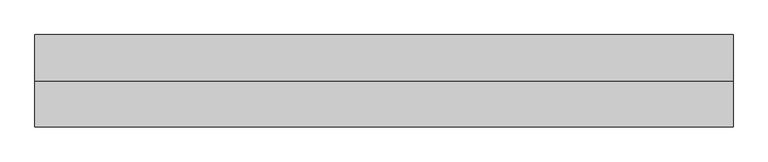
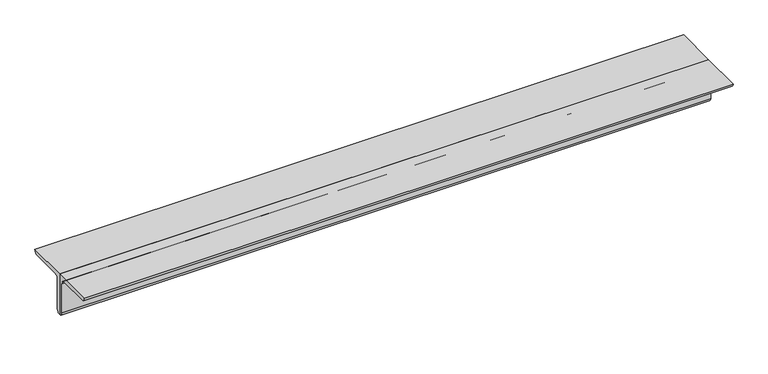
"""IFC4 building model written with IfcOpenShell, lengths in millimetres: beam geometry, 0123_Steel Framing_2Ls-KSD3502 : H_SB_AR_S04_2Ls-130x130x12_VBR1."""

from ifc_helpers import new_model, si_unit, point, frame, frame_2d, origin, place, context, project, spatial, polyline, circle_curve, trimmed, segment, composite_curve, outline, extrude, source, transform, mapped, element, save


def beam_0ae2001c(model_context):
    return source(origin(), model_context, "Body", "SweptSolid", [
        extrude(outline(composite_curve([segment(polyline([(0.0, 36.4), (130.0, 36.4)]), True, "CONTINUOUS"), segment(trimmed(circle_curve(frame_2d((118.0, 36.4)), 12.0), [point((130.0, 36.4))], [point((118.0, 24.4))], False, "CARTESIAN"), True, "CONTINUOUS"), segment(polyline([(118.0, 24.4), (24.0, 24.4)]), True, "CONTINUOUS"), segment(trimmed(circle_curve(frame_2d((24.0, 12.4)), 12.0), [point((24.0, 24.4))], [point((12.0, 12.4))], True, "CARTESIAN"), True, "CONTINUOUS"), segment(polyline([(12.0, 12.4), (12.0, -81.6)]), True, "CONTINUOUS"), segment(trimmed(circle_curve(frame_2d((0.0, -81.6)), 12.0), [point((12.0, -81.6))], [point((0.0, -93.6))], False, "CARTESIAN"), True, "CONTINUOUS"), segment(polyline([(0.0, -93.6), (0.0, 36.4)]), True, "CONTINUOUS")], self_intersect=False)), frame((-912.8215992, 0.0, 0.0), z_axis=(1.0, 0.0, 0.0), x_axis=(0.0, 1.0, 0.0)), (0.0, 0.0, 1.0), 1965.6424176),
        extrude(outline(composite_curve([segment(polyline([(0.0, 36.4), (0.0, -93.6)]), True, "CONTINUOUS"), segment(trimmed(circle_curve(frame_2d((0.0, -81.6)), 12.0), [point((0.0, -93.6))], [point((-12.0, -81.6))], False, "CARTESIAN"), True, "CONTINUOUS"), segment(polyline([(-12.0, -81.6), (-12.0, 12.4)]), True, "CONTINUOUS"), segment(trimmed(circle_curve(frame_2d((-24.0, 12.4)), 12.0), [point((-12.0, 12.4))], [point((-24.0, 24.4))], True, "CARTESIAN"), True, "CONTINUOUS"), segment(polyline([(-24.0, 24.4), (-118.0, 24.4)]), True, "CONTINUOUS"), segment(trimmed(circle_curve(frame_2d((-118.0, 36.4)), 12.0), [point((-118.0, 24.4))], [point((-130.0, 36.4))], False, "CARTESIAN"), True, "CONTINUOUS"), segment(polyline([(-130.0, 36.4), (0.0, 36.4)]), True, "CONTINUOUS")], self_intersect=False)), frame((-912.8215992, 0.0, 0.0), z_axis=(1.0, 0.0, 0.0), x_axis=(0.0, 1.0, 0.0)), (0.0, 0.0, 1.0), 1965.6424176),
    ])


if __name__ == "__main__":
    model = new_model("IFC4")
    model_context = context("Model", 3, world=origin())
    ifc_project = project(units=[si_unit("LENGTHUNIT", "METRE", prefix="MILLI")], contexts=[model_context])
    site = spatial("IfcSite", under=ifc_project)
    building = spatial("IfcBuilding", under=site)
    placement = place(None, origin())
    beam_shape = beam_0ae2001c(model_context)
    element("IfcBeam", 1, ObjectType="0123_Steel Framing_2Ls-KSD3502 : H_SB_AR_S04_2Ls-130x130x12_VBR1", at=placement, inside=building, context=model_context, shape_type="MappedRepresentation", body=[
        mapped(beam_shape, transform((0.0, 0.0, 0.0), x_axis=(1.0, 0.0, 0.0), y_axis=(0.0, 1.0, 0.0), z_axis=(0.0, 0.0, 1.0))),
    ])
    save(model, "model.ifc")

# Revit data of these elements
# Type "0123_Steel Framing_2Ls-KSD3502 : H_SB_AR_S04_2Ls-130x130x12_VBR1"
#   Type Mark = "VBR1"
#   Assembly Code = "B10"
#   Legs = "SLBB"
#   W = 8.97
#   Perimeter = 1.04 m²/m
#   Nominal Weight = 46.80 kgf/m
#   Length [instance default] = 1000 mm
#   Space = 0 mm
#   b = 130 mm
#   d = 130 mm
#   t = 12 mm
#   y = 36.4 mm
#   A = 0.005952 m²
#   Structural Material [instance default] = Steel ASTM A36
# Element 1 (IfcBeam, "0123_Steel Framing_2Ls-KSD3502 : H_SB_AR_S04_2Ls-130x130x12_VBR1")
#   Materials on its faces: "Steel ASTM A36"
# Materials
#   "Steel ASTM A36": class "Metal", colour RGB 199 199 199, transparency 0, Description = "Structural steel, ASTM A36 Grade B, mill finish", Cost = 0
